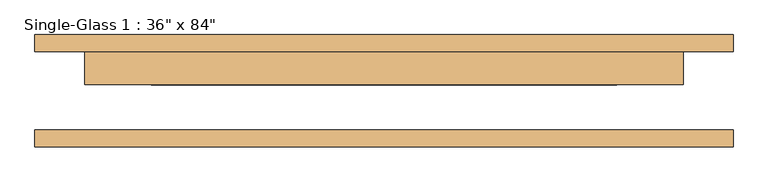
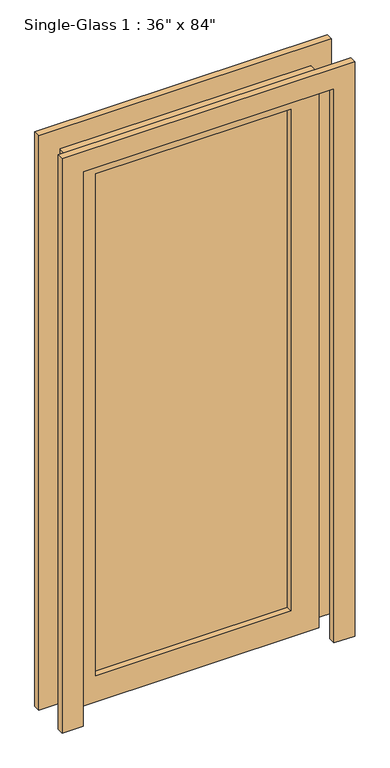
"""IFC4 building model written with IfcOpenShell, lengths in millimetres: door geometry."""

from ifc_helpers import new_model, si_unit, frame, origin, place, context, project, spatial, polyline, outline, extrude, source, transform, mapped, element, save


def door_e93cdbe7(model_context):
    return source(origin(), model_context, "Body", "SweptSolid", [
        extrude(outline(polyline([(2133.6, 457.2), (0.0, 457.2), (0.0, 533.4), (2209.8, 533.4), (2209.8, -533.4), (0.0, -533.4), (0.0, -457.2), (2133.6, -457.2), (2133.6, 457.2)])), frame((0.0, -85.725, 0.0), z_axis=(0.0, 1.0, 0.0), x_axis=(0.0, 0.0, 1.0)), (0.0, 0.0, 1.0), 25.4),
        extrude(outline(polyline([(2133.6, 457.2), (0.0, 457.2), (0.0, 533.4), (2209.8, 533.4), (2209.8, -533.4), (0.0, -533.4), (0.0, -457.2), (2133.6, -457.2), (2133.6, 457.2)])), frame((0.0, 60.325, 0.0), z_axis=(0.0, 1.0, 0.0), x_axis=(0.0, 0.0, 1.0)), (0.0, 0.0, 1.0), 25.4),
        extrude(outline(polyline([(355.6, 31.75), (-355.6, 31.75), (-355.6, 38.1), (355.6, 38.1), (355.6, 31.75)])), frame((0.0, 0.0, 101.6), z_axis=(0.0, 0.0, 1.0), x_axis=(1.0, 0.0, 0.0)), (0.0, 0.0, 1.0), 1930.4),
        extrude(outline(polyline([(2133.6, 457.2), (2133.6, -457.2), (0.0, -457.2), (0.0, 457.2), (2133.6, 457.2)]), holes=[polyline([(2032.0, -355.6), (2032.0, 355.6), (101.6, 355.6), (101.6, -355.6), (2032.0, -355.6)])]), frame((0.0, 9.525, 0.0), z_axis=(0.0, 1.0, 0.0), x_axis=(0.0, 0.0, 1.0)), (0.0, 0.0, 1.0), 50.8),
    ])


if __name__ == "__main__":
    model = new_model("IFC4")
    model_context = context("Model", 3, world=origin())
    ifc_project = project(units=[si_unit("LENGTHUNIT", "METRE", prefix="MILLI")], contexts=[model_context])
    site = spatial("IfcSite", under=ifc_project)
    building = spatial("IfcBuilding", under=site)
    placement = place(None, origin())
    door_shape = door_e93cdbe7(model_context)
    element("IfcDoor", 1, ObjectType="Single-Glass 1 : 36\" x 84\"", at=placement, inside=building, context=model_context, shape_type="MappedRepresentation", body=[
        mapped(door_shape, transform((0.0, 0.0, 0.0), x_axis=(1.0, 0.0, 0.0), y_axis=(0.0, 1.0, 0.0), z_axis=(0.0, 0.0, 1.0))),
    ])
    save(model, "model.ifc")

# Revit data of these elements
# Type "Single-Glass 1 : 36\" x 84\""
#   Type Mark = "20"
#   Construction Type Id = "MDOOR"
#   Assembly Code = "C1020"
#   Analytic Construction = "Metal"
#   Thickness = 0' - 2"
#   Heat Transfer Coefficient (U) = 3.7021 W/(m²·K)
#   Height = 7' - 0"
#   Rail Width - Base = 0' - 4"
#   Rail Width - Top = 0' - 4"
#   Stile Width - Hinge = 0' - 4"
#   Stile Width - Latch = 0' - 4"
#   Trim Projection Ext = 0' - 1"
#   Trim Projection Int = 0' - 1"
#   Trim Width = 0' - 3"
#   Width = 3' - 0"
#   Door Material = Aluminum
#   Frame Material = Aluminum
#   Visual Light Transmittance = 0
#   Solar Heat Gain Coefficient = 0
#   Function = (empty or 0)
#   Wall Closure = (empty or 0)
# Element 1 (IfcDoor, "Single-Glass 1 : 36\" x 84\"")
#   Materials on its faces: "Aluminum", "Glass"
# Materials
#   "Aluminum": class "Metal", colour RGB 226 226 226, transparency 0, Description = "Aluminum 6061", Cost = 0
#   "Glass": class "Glass", colour RGB 142 168 196, transparency 0.75, Description = "Soda Lime Glass", Cost = 0
